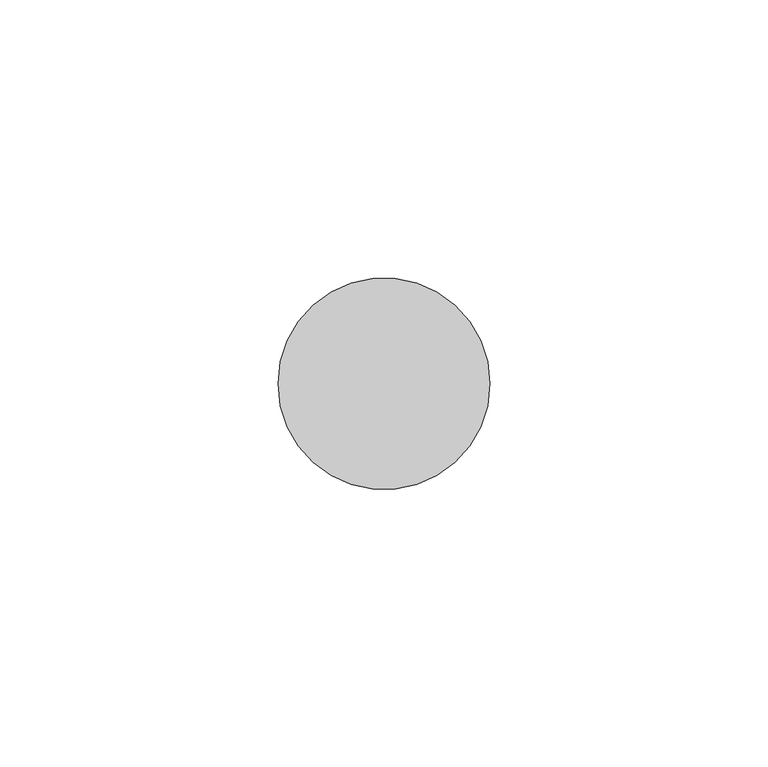
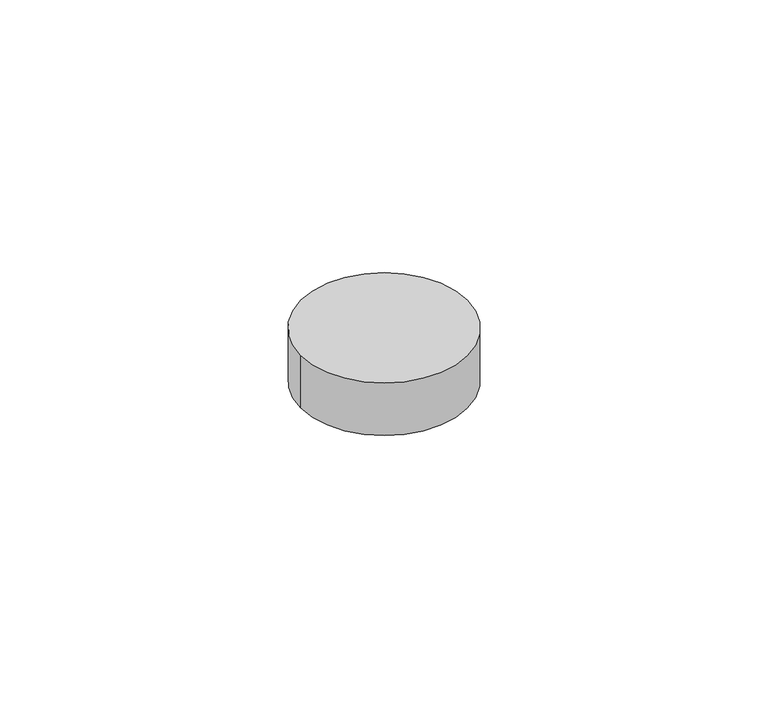
"""IFC4 building model written with IfcOpenShell, lengths in millimetres: proxy geometry, Bolt001 8681 : Bolt001 8681."""

from ifc_helpers import new_model, si_unit, point, frame, frame_2d, origin, place, context, project, spatial, circle_curve, trimmed, segment, composite_curve, outline, extrude, source, transform, mapped, element, save


def generic_models_70c8ac4d(model_context):
    return source(origin(), model_context, "Body", "SweptSolid", [
        extrude(outline(composite_curve([segment(trimmed(circle_curve(frame_2d((7251.9702148, -1781.8449707)), 19.05), [point((7232.9202148, -1781.8449707))], [point((7271.0202148, -1781.8449707))], False, "CARTESIAN"), True, "CONTINUOUS"), segment(trimmed(circle_curve(frame_2d((7251.9702148, -1781.8449707)), 19.05), [point((7271.0202148, -1781.8449707))], [point((7232.9202148, -1781.8449707))], False, "CARTESIAN"), True, "CONTINUOUS")], self_intersect=False)), frame((0.0, 0.0, 40112.696), z_axis=(0.0, 0.0, 1.0), x_axis=(1.0, 0.0, 0.0)), (0.0, 0.0, 1.0), 12.7),
    ])


if __name__ == "__main__":
    model = new_model("IFC4")
    model_context = context("Model", 3, world=origin())
    ifc_project = project(units=[si_unit("LENGTHUNIT", "METRE", prefix="MILLI")], contexts=[model_context])
    site = spatial("IfcSite", under=ifc_project)
    building = spatial("IfcBuilding", under=site)
    placement = place(None, origin())
    generic_models_shape = generic_models_70c8ac4d(model_context)
    element("IfcBuildingElementProxy", 1, Name="Bolt001 8681 : Bolt001 8681", ObjectType="Bolt001 8681 : Bolt001 8681", at=placement, inside=building, context=model_context, shape_type="MappedRepresentation", body=[
        mapped(generic_models_shape, transform((0.0, 0.0, 0.0), x_axis=(1.0, 0.0, 0.0), y_axis=(0.0, 1.0, 0.0), z_axis=(0.0, 0.0, 1.0))),
    ])
    save(model, "model.ifc")

# Revit data of these elements
# Type "Bolt001 8681 : Bolt001 8681"
#   NameOverride = "Bolt001"
# Element 1 (IfcBuildingElementProxy, "Bolt001 8681 : Bolt001 8681")
#   Materials on its faces: "BOLTS CONCEALED BY FLOOR FINISH"
# Materials
#   "BOLTS CONCEALED BY FLOOR FINISH": class "Unassigned", colour RGB 128 128 128, transparency 0
